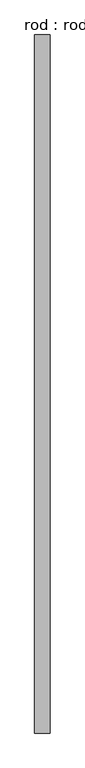
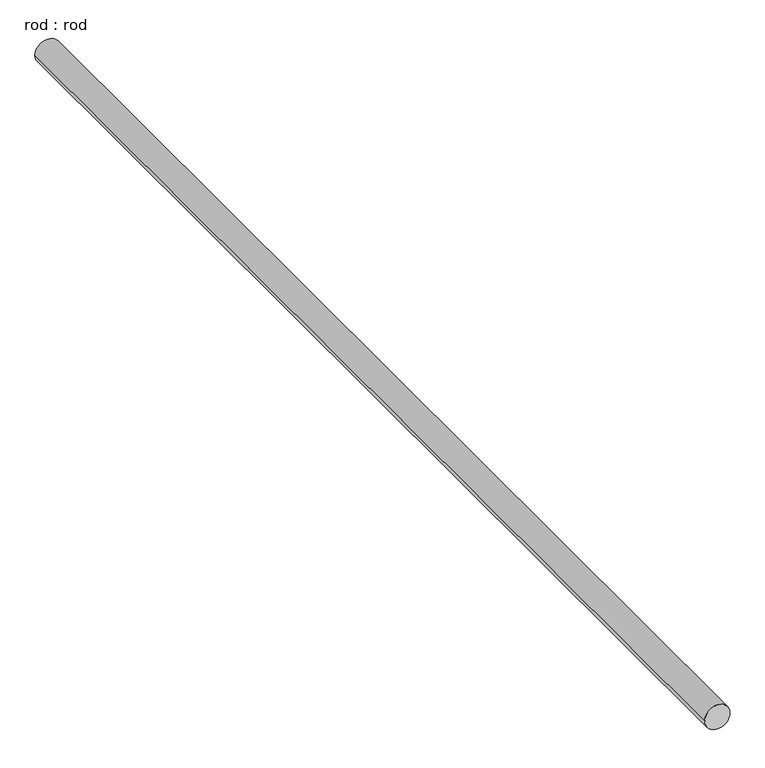
"""IFC4 building model written with IfcOpenShell, lengths in millimetres: proxy geometry, rod : rod."""

from ifc_helpers import new_model, si_unit, point, frame, frame_2d, origin, place, context, project, spatial, circle_curve, trimmed, segment, composite_curve, outline, extrude, source, transform, mapped, element, save


def rod_rod_5bb9b93d(model_context):
    return source(origin(), model_context, "Body", "SweptSolid", [
        extrude(outline(composite_curve([segment(trimmed(circle_curve(frame_2d((0.0108462, 0.0)), 200.0), [point((0.0108462, 200.0))], [point((0.0108462, -200.0))], False, "CARTESIAN"), True, "CONTINUOUS"), segment(trimmed(circle_curve(frame_2d((0.0108462, 0.0)), 200.0), [point((0.0108462, -200.0))], [point((0.0108462, 200.0))], False, "CARTESIAN"), True, "CONTINUOUS")], self_intersect=False)), frame((0.0, -5087.1041287, 0.0), z_axis=(0.0, 1.0, 0.0), x_axis=(0.0, 0.0, 1.0)), (0.0, 0.0, 1.0), 18359.6654881),
    ])


if __name__ == "__main__":
    model = new_model("IFC4")
    model_context = context("Model", 3, world=origin())
    ifc_project = project(units=[si_unit("LENGTHUNIT", "METRE", prefix="MILLI")], contexts=[model_context])
    site = spatial("IfcSite", under=ifc_project)
    building = spatial("IfcBuilding", under=site)
    placement = place(None, origin())
    rod_rod_shape = rod_rod_5bb9b93d(model_context)
    element("IfcBuildingElementProxy", 1, Name="rod : rod", ObjectType="rod : rod", at=placement, inside=building, context=model_context, shape_type="MappedRepresentation", body=[
        mapped(rod_rod_shape, transform((0.0, 0.0, 0.0), x_axis=(1.0, 0.0, 0.0), y_axis=(0.0, 1.0, 0.0), z_axis=(0.0, 0.0, 1.0))),
    ])
    save(model, "model.ifc")

# Revit data of these elements
# Type "rod : rod"
#   Default Elevation = 0
